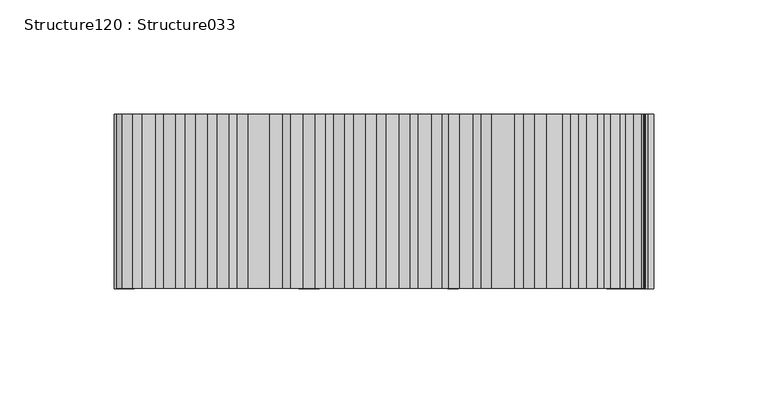
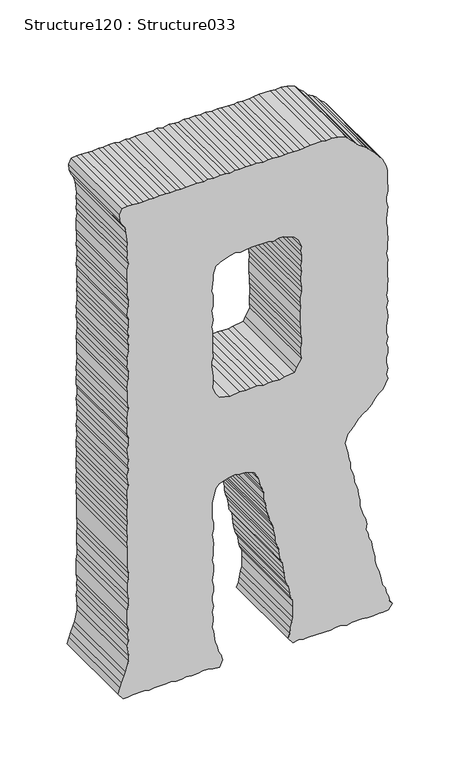
"""IFC4 building model written with IfcOpenShell, lengths in millimetres: proxy geometry, Structure120 : Structure033."""

import ifcopenshell
import ifcopenshell.guid

model = None  # the IFC model being written
_history = None  # IfcOwnerHistory: only IFC2X3 demands one
_inside = {}  # id of a spatial element -> (the spatial element, [elements in it])
_under = {}  # id of a project, library or spatial element -> (it, [spatial elements below it])
_declared = {}  # id of a project -> (the project, [libraries it declares])
_typed = {}  # id of a type object -> (the type object, [elements of that type])
_made_of = {}  # id of a material, layer set ... -> (it, [elements and type objects made of it])


def new_model(schema):
    """Start an empty IFC model of exactly this schema.

    Asked for "IFC4X3", IfcOpenShell would pick the latest addendum, in which some entities
    have other attributes; the version numbers below select the first issue.
    IFC2X3 requires an IfcOwnerHistory on every rooted entity: one is made here for all.
    """
    global model, _history
    if schema == "IFC4X3":
        model = ifcopenshell.file(schema_version=(4, 3, 0, 0))
    else:
        model = ifcopenshell.file(schema=schema)
    _inside.clear()
    _under.clear()
    _declared.clear()
    _typed.clear()
    _made_of.clear()
    _history = None
    if model.schema == "IFC2X3":
        org = make("IfcOrganization", Name="unknown")
        user = make(
            "IfcPersonAndOrganization",
            ThePerson=make("IfcPerson", FamilyName="unknown"),
            TheOrganization=org,
        )
        app = make(
            "IfcApplication",
            ApplicationDeveloper=org,
            Version="unknown",
            ApplicationFullName="unknown",
            ApplicationIdentifier="unknown",
        )
        _history = make(
            "IfcOwnerHistory",
            OwningUser=user,
            OwningApplication=app,
            ChangeAction="ADDED",
            CreationDate=0,
        )
    return model


def make(cls, **values):
    """One entity of the class cls with the attributes given. An attribute that is None is left unset."""
    return model.create_entity(
        cls, **{name: value for name, value in values.items() if value is not None}
    )


def rooted(cls, **values):
    """An entity with a GlobalId (a new one), such as an element, a storey or a relation."""
    return make(cls, GlobalId=ifcopenshell.guid.new(), OwnerHistory=_history, **values)


def si_unit(unit_type, name, prefix=None):
    """IfcSIUnit, for example si_unit("LENGTHUNIT", "METRE", prefix="MILLI")."""
    return make("IfcSIUnit", UnitType=unit_type, Prefix=prefix, Name=name)


def assignment(units):
    """IfcUnitAssignment: the units of a project."""
    return None if units is None else make("IfcUnitAssignment", Units=units)


def point(xyz):
    """IfcCartesianPoint."""
    return None if xyz is None else make("IfcCartesianPoint", Coordinates=xyz)


def direction(xyz):
    """IfcDirection."""
    return None if xyz is None else make("IfcDirection", DirectionRatios=xyz)


def frame(location, z_axis=None, x_axis=None):
    """IfcAxis2Placement3D, a coordinate frame: its origin and axes. An axis left out is left unset."""
    return make(
        "IfcAxis2Placement3D",
        Location=point(location),
        Axis=direction(z_axis),
        RefDirection=direction(x_axis),
    )


def origin():
    """The frame at (0, 0, 0) with its axes left unset."""
    return frame((0.0, 0.0, 0.0))


def place(relative_to, where):
    """IfcLocalPlacement: puts the frame where relative to a parent placement (None: the world)."""
    return make(
        "IfcLocalPlacement", PlacementRelTo=relative_to, RelativePlacement=where
    )


def context(
    kind, dimensions, precision=None, world=None, true_north=None, identifier=None
):
    """IfcGeometricRepresentationContext, for example the 3D "Model" context."""
    return make(
        "IfcGeometricRepresentationContext",
        ContextIdentifier=identifier,
        ContextType=kind,
        CoordinateSpaceDimension=dimensions,
        Precision=precision,
        WorldCoordinateSystem=world,
        TrueNorth=true_north,
    )


def project(units=None, contexts=None):
    """IfcProject with its units and contexts."""
    return rooted(
        "IfcProject",
        Name="project",
        RepresentationContexts=contexts,
        UnitsInContext=assignment(units),
    )


def spatial(cls, under=None, at=None, **own):
    """A site, building, storey or space (cls), placed at a placement, below another one or the project."""
    s = rooted(cls, ObjectPlacement=at, **own)
    if under is not None:
        _under.setdefault(under.id(), (under, []))[1].append(s)
    return s


def polyline(points):
    """IfcPolyline through the points."""
    return make("IfcPolyline", Points=[point(p) for p in points])


def outline(outer, holes=None, kind="AREA"):
    """IfcArbitraryClosedProfileDef: a profile drawn as a closed curve; with holes, ...WithVoids."""
    if holes is None:
        return make("IfcArbitraryClosedProfileDef", ProfileType=kind, OuterCurve=outer)
    return make(
        "IfcArbitraryProfileDefWithVoids",
        ProfileType=kind,
        OuterCurve=outer,
        InnerCurves=holes,
    )


def extrude(swept, where, along, depth):
    """IfcExtrudedAreaSolid: the profile swept, set in the frame where, extruded along a direction by depth."""
    return make(
        "IfcExtrudedAreaSolid",
        SweptArea=swept,
        Position=where,
        ExtrudedDirection=direction(along),
        Depth=depth,
    )


def shape(context_of_items, identifier, shape_type, items):
    """IfcShapeRepresentation: the items that make up one representation, for example the "Body"."""
    return make(
        "IfcShapeRepresentation",
        ContextOfItems=context_of_items,
        RepresentationIdentifier=identifier,
        RepresentationType=shape_type,
        Items=items,
    )


def source(mapping_origin, context_of_items, identifier, shape_type, items):
    """IfcRepresentationMap: a shape defined once, which mapped items show again and again."""
    return make(
        "IfcRepresentationMap",
        MappingOrigin=mapping_origin,
        MappedRepresentation=shape(context_of_items, identifier, shape_type, items),
    )


def transform(
    local_origin,
    x_axis=None,
    y_axis=None,
    z_axis=None,
    scale=None,
    scale2=None,
    scale3=None,
    uniform=True,
):
    """IfcCartesianTransformationOperator3D, or its non-uniform kind. x_axis, y_axis, z_axis: its Axis1, 2, 3."""
    if uniform:
        return make(
            "IfcCartesianTransformationOperator3D",
            Axis1=direction(x_axis),
            Axis2=direction(y_axis),
            LocalOrigin=point(local_origin),
            Scale=scale,
            Axis3=direction(z_axis),
        )
    return make(
        "IfcCartesianTransformationOperator3DnonUniform",
        Axis1=direction(x_axis),
        Axis2=direction(y_axis),
        LocalOrigin=point(local_origin),
        Scale=scale,
        Axis3=direction(z_axis),
        Scale2=scale2,
        Scale3=scale3,
    )


def mapped(mapping_source, mapping_target):
    """IfcMappedItem: shows the shape of a source again, moved by a transform."""
    return make(
        "IfcMappedItem", MappingSource=mapping_source, MappingTarget=mapping_target
    )


def made_of(thing, what):
    """Note that an element or type object is made of a material, layer set ...; save() writes the relation."""
    if what is not None:
        _made_of.setdefault(what.id(), (what, []))[1].append(thing)
    return thing


def element(
    cls,
    number,
    at=None,
    inside=None,
    cuts=None,
    type_object=None,
    material=None,
    context=None,
    identifier="Body",
    shape_type=None,
    held_by="IfcProductDefinitionShape",
    body=None,
    shapes=None,
    **own,
):
    """One element of the class cls, such as IfcWall. Its Tag is "e" and its number.

    at: its placement. inside: the storey or other place that contains it. cuts: it is an
    opening in that element (IfcRelVoidsElement). A single representation is given by context,
    identifier, shape_type and body (its items); several are given by shapes. held_by: the class
    of the entity that holds the representations. save() writes the other relations.
    """
    e = rooted(cls, Tag="e%d" % number, ObjectPlacement=at, **own)
    if body is not None:
        shapes = [shape(context, identifier, shape_type, body)]
    if shapes is not None:
        e.Representation = make(held_by, Representations=shapes)
    if inside is not None:
        _inside.setdefault(inside.id(), (inside, []))[1].append(e)
    if cuts is not None:
        rooted(
            "IfcRelVoidsElement", RelatingBuildingElement=cuts, RelatedOpeningElement=e
        )
    if type_object is not None:
        _typed.setdefault(type_object.id(), (type_object, []))[1].append(e)
    return made_of(e, material)


def aggregate(whole, parts):
    """IfcRelAggregates: a whole, such as a stair, and the parts it consists of."""
    return rooted("IfcRelAggregates", RelatingObject=whole, RelatedObjects=parts)


def save(model, path):
    """Write the relations noted so far, then the file.

    IfcRelAggregates (storeys below a building ...), IfcRelContainedInSpatialStructure (elements
    in a storey), IfcRelDefinesByType, IfcRelAssociatesMaterial and IfcRelDeclares: one each for
    every whole, place, type object, material and project.
    """
    for whole, parts in _under.values():
        aggregate(whole, parts)
    for where, things in _inside.values():
        rooted(
            "IfcRelContainedInSpatialStructure",
            RelatedElements=things,
            RelatingStructure=where,
        )
    for kind, things in _typed.values():
        rooted("IfcRelDefinesByType", RelatedObjects=things, RelatingType=kind)
    for what, things in _made_of.values():
        rooted("IfcRelAssociatesMaterial", RelatedObjects=things, RelatingMaterial=what)
    for by, libraries in _declared.values():
        rooted("IfcRelDeclares", RelatingContext=by, RelatedDefinitions=libraries)
    model.write(path)


def structure120_structure033_93d3bff6(model_context):
    return source(origin(), model_context, "Body", "SweptSolid", [
        extrude(outline(polyline([(3899.7046941, -39455.6190419), (3903.2059411, -39456.2207686), (3907.888177, -39456.2207686), (3918.4480792, -39455.0397797), (3923.1319197, -39456.2207686), (3927.8077372, -39456.2207686), (3932.4899731, -39455.0397797), (3936.0345445, -39455.0397797), (3941.8753048, -39455.6190419), (3951.2606365, -39455.6190419), (3955.360401, -39456.2207686), (3962.9774586, -39459.7188064), (3967.6789497, -39463.2409133), (3970.5768654, -39465.5804266), (3974.1214368, -39469.6817957), (3977.6194746, -39472.6230357), (3979.9621971, -39475.5418113), (3982.8793681, -39480.2449071), (3987.0048063, -39483.7445495), (3989.9460463, -39487.2650518), (3994.0233463, -39490.7646942), (3996.390138, -39497.8056987), (3997.5486624, -39503.0880567), (3996.9645864, -39507.768688), (3997.5486624, -39511.8684525), (3997.5486624, -39521.8314418), (3996.9645864, -39526.532933), (3996.390138, -39530.0325754), (3996.390138, -39535.8941956), (3996.9645864, -39540.5956868), (3996.390138, -39543.516067), (3996.390138, -39548.1950937), (3996.9645864, -39554.0567139), (3996.9645864, -39557.5563563), (3996.390138, -39562.2578475), (3997.5486624, -39568.1194677), (3996.9645864, -39572.2192322), (3997.5486624, -39576.922328), (3996.9645864, -39582.1822215), (3997.5486624, -39586.281986), (3996.390138, -39590.9626173), (3996.9645864, -39594.4831196), (3997.5486624, -39599.1862153), (3996.390138, -39604.4461089), (3997.5486624, -39609.7060024), (3996.390138, -39613.2265047), (3996.9645864, -39619.0881249), (3996.9645864, -39628.4702474), (3996.390138, -39633.1508787), (3996.9645864, -39636.671381), (3996.390138, -39641.953739), (3996.9645864, -39646.0535035), (3996.9645864, -39651.313397), (3996.390138, -39655.9940283), (3996.9645864, -39660.1162573), (3996.390138, -39665.3761508), (3996.390138, -39668.8966531), (3996.9645864, -39674.7582733), (3996.9645864, -39678.8596424), (3996.390138, -39683.5611335), (3991.6806238, -39685.879787), (3986.4046842, -39685.3005248), (3981.7208437, -39683.5611335), (3978.2035506, -39681.1991557), (3973.5197101, -39680.0406313), (3963.5615346, -39678.8596424), (3959.4617701, -39679.4389046), (3954.7506513, -39678.8596424), (3949.4923624, -39679.4389046), (3944.8165449, -39678.2579157), (3939.5325823, -39679.4389046), (3930.1745289, -39679.4389046), (3926.6492128, -39678.8596424), (3920.7908018, -39678.8596424), (3916.0909152, -39679.4389046), (3911.4054701, -39678.2579157), (3906.7328618, -39678.2579157), (3903.2059411, -39678.8596424), (3897.3475301, -39679.4389046), (3893.822214, -39678.2579157), (3887.9621984, -39678.2579157), (3883.2863809, -39678.8596424), (3878.5784713, -39678.2579157), (3875.0772243, -39678.8596424), (3870.4030114, -39678.2579157), (3865.7015202, -39678.2579157), (3859.8591552, -39679.4389046), (3855.7353217, -39678.8596424), (3850.4754282, -39679.4389046), (3846.3772683, -39678.2579157), (3841.0900965, -39678.2579157), (3836.9919366, -39678.8596424), (3831.732043, -39679.4389046), (3828.2163546, -39678.8596424), (3818.2309008, -39678.8596424), (3812.9726119, -39678.2579157), (3809.4729695, -39678.8596424), (3803.5872802, -39679.4389046), (3798.9050443, -39678.8596424), (3794.8309535, -39679.4389046), (3789.5293402, -39679.4389046), (3786.0280932, -39678.2579157), (3780.1616592, -39678.2579157), (3776.6427615, -39679.4389046), (3771.9605256, -39678.8596424), (3766.1021146, -39678.2579157), (3761.418274, -39678.8596424), (3757.8753073, -39678.2579157), (3752.6170184, -39679.4389046), (3747.9428055, -39678.8596424), (3742.6748889, -39678.2579157), (3738.5574738, -39679.4389046), (3733.2991849, -39679.4389046), (3729.1737467, -39678.8596424), (3725.0996559, -39678.8596424), (3720.4158154, -39679.4389046), (3714.5301261, -39679.4389046), (3709.8559132, -39678.8596424), (3706.3289925, -39679.4389046), (3701.6547796, -39679.4389046), (3695.786741, -39678.8596424), (3691.0868544, -39679.4389046), (3686.4030139, -39678.8596424), (3668.2437048, -39678.8596424), (3663.5598643, -39678.2579157), (3658.8840468, -39678.2579157), (3654.1841602, -39678.8596424), (3645.4262289, -39678.8596424), (3639.5405396, -39678.2579157), (3634.856699, -39678.2579157), (3630.1824862, -39679.4389046), (3616.69739, -39679.4389046), (3612.0135494, -39678.2579157), (3607.8961343, -39678.8596424), (3602.0280957, -39678.2579157), (3597.9540049, -39679.4389046), (3588.5702778, -39678.2579157), (3583.8864372, -39678.2579157), (3574.5107332, -39680.6198935), (3570.9854171, -39681.8008824), (3565.7094775, -39684.1403958), (3561.6257591, -39685.3005248), (3556.3417965, -39687.0607759), (3551.0658569, -39682.9594069), (3551.0658569, -39678.8596424), (3551.6675836, -39674.7582733), (3551.6675836, -39664.7968886), (3551.0658569, -39660.6955195), (3551.6675836, -39655.9940283), (3551.6675836, -39646.0535035), (3552.242032, -39641.3520123), (3551.0658569, -39637.2731077), (3551.0658569, -39632.5716165), (3551.6675836, -39628.4702474), (3551.0658569, -39623.7896161), (3551.6675836, -39618.5088627), (3552.242032, -39614.4074936), (3552.242032, -39610.3077291), (3551.0658569, -39605.6270978), (3550.4833855, -39599.7654776), (3556.3417965, -39597.4034997), (3561.6257591, -39598.5844887), (3565.1254015, -39600.9464665), (3570.9854171, -39602.0841311), (3574.5107332, -39603.8668467), (3585.0706354, -39605.0253711), (3589.1527492, -39606.20636), (3594.4286888, -39605.6270978), (3597.9540049, -39605.6270978), (3602.6298224, -39606.20636), (3607.8961343, -39605.0253711), (3613.1720739, -39606.20636), (3617.2718384, -39606.20636), (3621.3732075, -39605.0253711), (3626.0554434, -39605.0253711), (3631.915459, -39606.20636), (3636.6153456, -39605.6270978), (3640.114988, -39605.0253711), (3644.8245022, -39605.0253711), (3650.1004418, -39606.20636), (3654.1841602, -39605.6270978), (3660.0682449, -39605.6270978), (3664.7440624, -39605.0253711), (3668.2437048, -39605.6270978), (3672.9435914, -39606.20636), (3677.6274319, -39605.0253711), (3683.4858429, -39605.0253711), (3688.1873341, -39606.20636), (3701.6547796, -39606.20636), (3706.9130685, -39605.0253711), (3713.9556777, -39603.26512), (3717.4729707, -39600.3447398), (3719.8140887, -39592.1436062), (3720.9726131, -39586.281986), (3719.8140887, -39582.7614837), (3719.8140887, -39576.922328), (3716.8985223, -39569.8797188), (3709.2718371, -39565.7799543), (3703.4134261, -39564.5973608), (3698.711935, -39562.8595742), (3695.2122926, -39561.6785853), (3689.3458585, -39561.6785853), (3685.2444894, -39560.4975963), (3679.9701544, -39559.3166074), (3675.8687854, -39558.7373452), (3670.5848228, -39556.9754895), (3667.0851803, -39555.816965), (3662.3836892, -39554.0567139), (3657.7014533, -39552.875725), (3652.4431643, -39551.7172005), (3648.3161216, -39551.7172005), (3644.2420307, -39550.5362116), (3639.5405396, -39548.7968204), (3634.856699, -39548.1950937), (3629.5984101, -39547.6158315), (3625.472972, -39545.2763181), (3620.7971545, -39544.6745914), (3616.0972679, -39544.0953292), (3611.4134274, -39543.516067), (3606.1551384, -39542.3334735), (3602.0280957, -39539.9939601), (3596.7698067, -39539.4146979), (3592.6700423, -39538.8354357), (3588.5702778, -39536.4734578), (3583.2863152, -39536.4734578), (3573.9266571, -39536.4734578), (3570.4109687, -39537.6544467), (3565.1254015, -39538.8354357), (3560.441561, -39539.4146979), (3556.3417965, -39541.174949), (3550.4833855, -39536.4734578), (3551.6675836, -39531.7928265), (3550.4833855, -39527.6914574), (3551.0658569, -39523.5916929), (3551.0658569, -39510.1082014), (3550.4833855, -39504.2465811), (3551.6675836, -39499.5675544), (3551.6675836, -39496.067912), (3550.4833855, -39490.1838273), (3551.6675836, -39486.0840629), (3551.6675836, -39477.3036671), (3551.0658569, -39472.6230357), (3551.0658569, -39467.3406777), (3551.6675836, -39462.661651), (3551.0658569, -39459.1395442), (3551.6675836, -39454.438053), (3556.3417965, -39450.9384106), (3559.2669905, -39453.2779239), (3564.54293, -39454.438053), (3568.0682461, -39456.2207686), (3572.7440636, -39457.379293), (3576.2693797, -39459.7188064), (3585.0706354, -39461.4806621), (3590.3289243, -39462.661651), (3595.5872132, -39465.0011644), (3600.2967274, -39466.1821533), (3604.3964919, -39466.1821533), (3609.6547808, -39467.3406777), (3613.772196, -39468.5008068), (3619.0385079, -39469.1025335), (3622.555801, -39471.4420468), (3627.8397636, -39472.0213091), (3631.3410106, -39473.8040247), (3636.6153456, -39473.202298), (3641.8832621, -39474.3608224), (3646.557475, -39476.7019404), (3654.7842823, -39479.0639182), (3660.6250426, -39479.0639182), (3665.3265338, -39480.2449071), (3670.0007467, -39480.8241693), (3674.1277895, -39481.9826938), (3678.2018803, -39483.7445495), (3683.4858429, -39484.3238117), (3687.587212, -39485.5048006), (3691.6869765, -39487.2650518), (3696.9709391, -39487.2650518), (3701.0723082, -39488.4460407), (3706.9130685, -39489.6045651), (3716.2887726, -39491.9456831), (3723.9154578, -39489.6045651), (3726.2742264, -39486.6857895), (3729.7738688, -39483.7445495), (3734.47536, -39480.2449071), (3737.9750024, -39476.1226782), (3739.7416719, -39473.202298), (3743.2332913, -39469.1025335), (3747.9428055, -39466.1821533), (3751.4424479, -39463.2409133), (3753.8012165, -39459.1395442), (3762.5848215, -39455.0397797), (3766.684586, -39456.2207686), (3771.3860772, -39455.0397797), (3777.2444882, -39456.2207686), (3781.9299333, -39456.2207686), (3785.4456218, -39455.0397797), (3790.7039107, -39455.0397797), (3794.8309535, -39456.2207686), (3800.0876378, -39455.0397797), (3804.1890069, -39456.2207686), (3810.0474179, -39456.2207686), (3818.2309008, -39455.0397797), (3823.5341187, -39455.6190419), (3827.6162325, -39456.2207686), (3832.8921721, -39455.0397797), (3838.1761347, -39456.2207686), (3842.8583706, -39455.6190419), (3846.9757858, -39455.6190419), (3851.6612309, -39455.0397797), (3856.9179152, -39455.6190419), (3866.8776953, -39455.6190419), (3870.4030114, -39455.0397797), (3876.263027, -39456.2207686), (3880.3627915, -39455.6190419), (3884.4609514, -39455.6190419), (3890.320967, -39455.0397797), (3894.4030808, -39455.6190419), (3899.7046941, -39455.6190419)]), holes=[polyline([(3794.8309535, -39582.7614837), (3793.6451507, -39590.9626173), (3795.960595, -39599.7654776), (3800.0876378, -39602.6858577), (3805.9476534, -39605.6270978), (3811.7884138, -39605.0253711), (3816.4883003, -39605.0253711), (3820.5896694, -39605.6270978), (3825.849563, -39606.20636), (3830.5574726, -39606.20636), (3834.6588416, -39605.0253711), (3839.9331766, -39605.6270978), (3858.1021133, -39605.6270978), (3861.6178018, -39606.20636), (3867.4601667, -39605.0253711), (3871.5599312, -39605.6270978), (3876.8438938, -39606.20636), (3880.3627915, -39605.0253711), (3890.320967, -39605.0253711), (3894.4030808, -39606.20636), (3904.9645876, -39605.0253711), (3909.0627475, -39605.0253711), (3916.0909152, -39602.6858577), (3918.4480792, -39599.1862153), (3921.3748778, -39590.9626173), (3922.5494483, -39586.281986), (3921.3748778, -39581.6029593), (3921.9733953, -39578.0808524), (3922.5494483, -39572.2192322), (3922.5494483, -39557.5563563), (3921.3748778, -39552.875725), (3922.5494483, -39549.3536181), (3922.5494483, -39544.6745914), (3919.0321552, -39535.8941956), (3915.5068392, -39532.3945532), (3908.46423, -39529.4533132), (3904.3901392, -39530.0325754), (3900.2887701, -39529.4533132), (3895.0048075, -39529.4533132), (3890.905043, -39530.0325754), (3885.6210804, -39529.4533132), (3880.9452629, -39530.0325754), (3876.8438938, -39530.0325754), (3871.5599312, -39529.4533132), (3867.4601667, -39529.4533132), (3862.2018778, -39530.6118376), (3858.1021133, -39530.6118376), (3854.0007442, -39530.0325754), (3849.3008577, -39530.6118376), (3839.9331766, -39530.6118376), (3834.0474873, -39530.0325754), (3829.374879, -39530.0325754), (3825.2911606, -39529.4533132), (3820.015221, -39529.4533132), (3816.4883003, -39530.0325754), (3810.6298893, -39530.0325754), (3806.5317294, -39529.4533132), (3800.0876378, -39533.5530777), (3795.960595, -39535.2924689), (3794.8309535, -39544.0953292), (3793.6451507, -39548.1950937), (3794.2292268, -39554.0567139), (3794.2292268, -39557.5563563), (3793.6451507, -39562.2578475), (3794.8309535, -39567.5402055), (3794.8309535, -39573.3793612), (3794.2292268, -39576.922328), (3794.8309535, -39582.7614837)])]), frame((0.0, 247945.1599557, 0.0), z_axis=(0.0, 1.0, 0.0), x_axis=(0.0, 0.0, 1.0)), (0.0, 0.0, 1.0), 76.2),
    ])


if __name__ == "__main__":
    model = new_model("IFC4")
    model_context = context("Model", 3, world=origin())
    ifc_project = project(units=[si_unit("LENGTHUNIT", "METRE", prefix="MILLI")], contexts=[model_context])
    site = spatial("IfcSite", under=ifc_project)
    building = spatial("IfcBuilding", under=site)
    placement = place(None, origin())
    structure120_structure033_shape = structure120_structure033_93d3bff6(model_context)
    element("IfcBuildingElementProxy", 1, Name="Structure120 : Structure033", ObjectType="Structure120 : Structure033", at=placement, inside=building, context=model_context, shape_type="MappedRepresentation", body=[
        mapped(structure120_structure033_shape, transform((0.0, 0.0, 0.0), x_axis=(1.0, 0.0, 0.0), y_axis=(0.0, 1.0, 0.0), z_axis=(0.0, 0.0, 1.0))),
    ])
    save(model, "model.ifc")

# Revit data of these elements
# Type "Structure120 : Structure033"
#   NameOverride = "Structure033"
# Element 1 (IfcBuildingElementProxy, "Structure120 : Structure033")
#   Materials on its faces: "BRUSHED ALUM. LETTERING"
# Materials
#   "BRUSHED ALUM. LETTERING": class "Unassigned", colour RGB 169 181 186, transparency 0, Cost = 0
